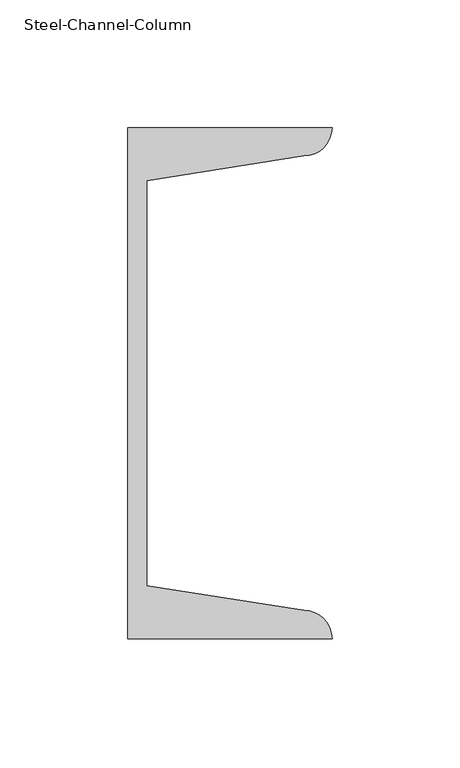
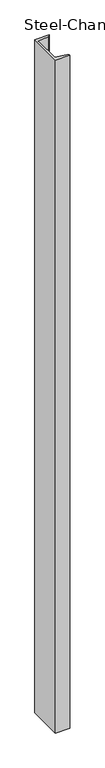
"""IFC4 building model written with IfcOpenShell, lengths in millimetres: column geometry, Steel-Channel-Column : CL126_C-200×80x7.5x11."""

from ifc_helpers import new_model, si_unit, point, frame_2d, origin, origin_with_axes, place, context, project, spatial, polyline, circle_curve, trimmed, segment, composite_curve, outline, extrude, source, transform, mapped, element, save


def steel_channel_column_727a91eb(model_context):
    return source(origin(), model_context, "Body", "SweptSolid", [
        extrude(outline(composite_curve([segment(polyline([(-22.1, -100.0), (-22.1, 100.0), (57.9, 100.0)]), True, "CONTINUOUS"), segment(trimmed(circle_curve(frame_2d((46.9, 100.0)), 11.0), [point((57.9, 100.0))], [point((46.9, 89.0))], False, "CARTESIAN"), True, "CONTINUOUS"), segment(polyline([(46.9, 89.0), (-14.6, 79.2593569), (-14.6, -79.2593569), (46.9, -89.0)]), True, "CONTINUOUS"), segment(trimmed(circle_curve(frame_2d((46.9, -100.0)), 11.0), [point((46.9, -89.0))], [point((57.9, -100.0))], False, "CARTESIAN"), True, "CONTINUOUS"), segment(polyline([(57.9, -100.0), (-22.1, -100.0)]), True, "CONTINUOUS")], self_intersect=False)), origin_with_axes(), (0.0, 0.0, 1.0), 4000.0),
    ])


if __name__ == "__main__":
    model = new_model("IFC4")
    model_context = context("Model", 3, world=origin())
    ifc_project = project(units=[si_unit("LENGTHUNIT", "METRE", prefix="MILLI")], contexts=[model_context])
    site = spatial("IfcSite", under=ifc_project)
    building = spatial("IfcBuilding", under=site)
    placement = place(None, origin())
    steel_channel_column_shape = steel_channel_column_727a91eb(model_context)
    element("IfcColumn", 1, ObjectType="Steel-Channel-Column : CL126_C-200×80x7.5x11", at=placement, inside=building, context=model_context, shape_type="MappedRepresentation", body=[
        mapped(steel_channel_column_shape, transform((0.0, 0.0, 0.0), x_axis=(1.0, 0.0, 0.0), y_axis=(0.0, 1.0, 0.0), z_axis=(0.0, 0.0, 1.0))),
    ])
    save(model, "model.ifc")

# Revit data of these elements
# Type "Steel-Channel-Column : CL126_C-200×80x7.5x11"
#   Assembly Code = "B10"
#   x = 22.1 mm
#   Section Area = 31.33 cm²
#   Mass per Unit Length = 24.60 kg/m
#   bf = 80 mm
#   d = 200 mm
#   tf = 11 mm
#   tw = 7.5 mm
#   hec_material4 [instance default] = none
#   hec_material3 [instance default] = none
#   hec_material2 [instance default] = none
#   hec_material1 [instance default] = none
#   Structural Material [instance default] = Steel, 45-345
# Element 1 (IfcColumn, "Steel-Channel-Column : CL126_C-200×80x7.5x11")
#   Materials on its faces: "Steel, 45-345"
# Materials
#   "Steel, 45-345": class "Metal", colour RGB 189 187 185, transparency 0, Description = "Steel 345 MPa", Cost = 0
